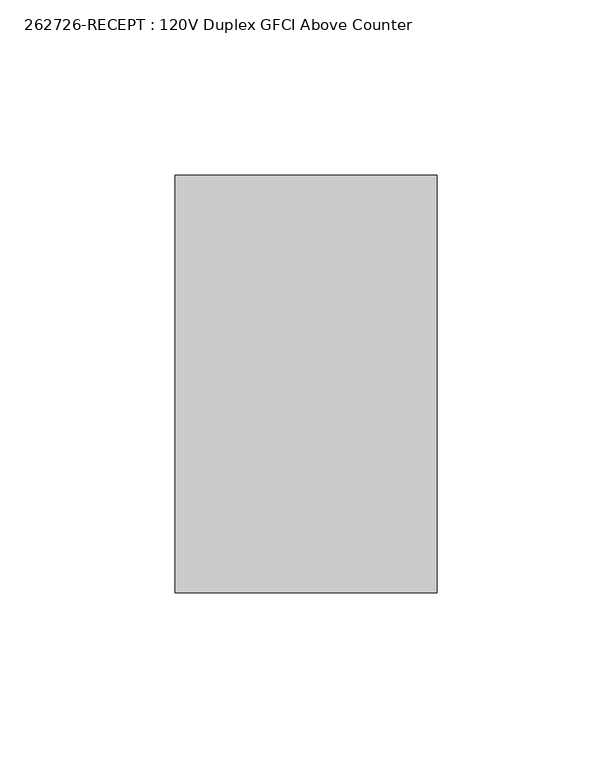
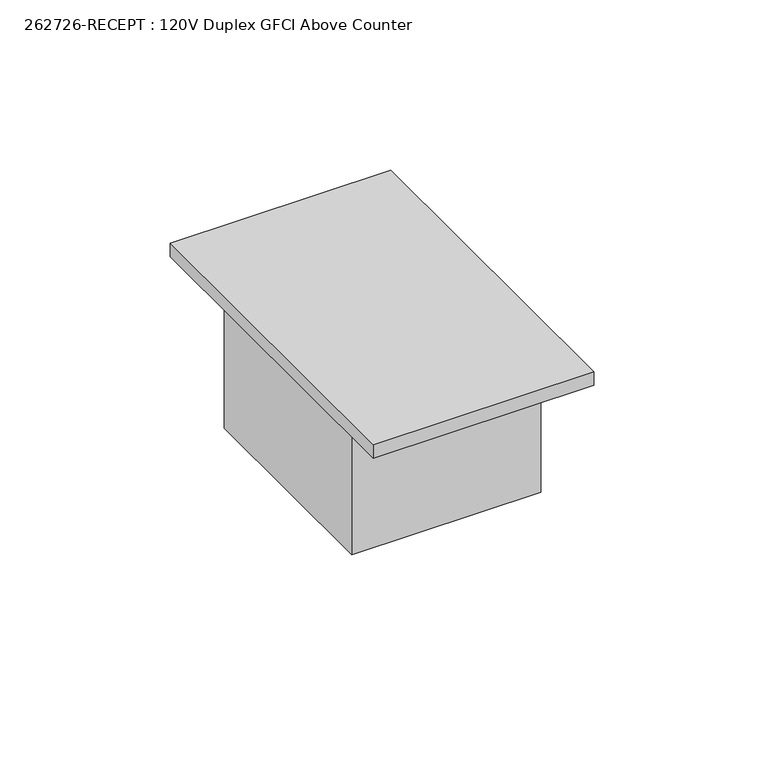
"""IFC4 building model written with IfcOpenShell, lengths in millimetres: proxy geometry, 262726-RECEPT : 120V Duplex GFCI Above Counter."""

from ifc_helpers import new_model, si_unit, frame, origin, origin_with_axes, place, context, project, spatial, polyline, outline, extrude, source, transform, mapped, element, save


def proxy_262726_recept_120v_duplex_gfci_above_counter_148ccacc(model_context):
    return source(origin(), model_context, "Body", "SweptSolid", [
        extrude(outline(polyline([(15.7308594, 59.5808594), (15.7308594, -59.5808594), (-58.9808594, -59.5808594), (-58.9808594, 59.5808594), (15.7308594, 59.5808594)])), origin_with_axes(), (0.0, 0.0, 1.0), 4.7625),
        extrude(outline(polyline([(10.5191406, 37.5), (10.5191406, -37.5), (-53.4808594, -37.5), (-53.4808594, 37.5), (10.5191406, 37.5)])), frame((0.0, 0.0, -50.0), z_axis=(0.0, 0.0, 1.0), x_axis=(1.0, 0.0, 0.0)), (0.0, 0.0, 1.0), 50.0),
    ])


if __name__ == "__main__":
    model = new_model("IFC4")
    model_context = context("Model", 3, world=origin())
    ifc_project = project(units=[si_unit("LENGTHUNIT", "METRE", prefix="MILLI")], contexts=[model_context])
    site = spatial("IfcSite", under=ifc_project)
    building = spatial("IfcBuilding", under=site)
    placement = place(None, origin())
    proxy_262726_recept_120v_duplex_gfci_above_counter_shape = proxy_262726_recept_120v_duplex_gfci_above_counter_148ccacc(model_context)
    element("IfcBuildingElementProxy", 1, Name="262726-RECEPT : 120V Duplex GFCI Above Counter", ObjectType="262726-RECEPT : 120V Duplex GFCI Above Counter", at=placement, inside=building, context=model_context, shape_type="MappedRepresentation", body=[
        mapped(proxy_262726_recept_120v_duplex_gfci_above_counter_shape, transform((0.0, 0.0, 0.0), x_axis=(1.0, 0.0, 0.0), y_axis=(0.0, 1.0, 0.0), z_axis=(0.0, 0.0, 1.0))),
    ])
    save(model, "model.ifc")

# Revit data of these elements
# Project information
#   Building Name = "RE1"
#   Client Name = "Client Name"
#   Project Address = "Project Address On One Line"
#   Project Name = "PROJECT NAME"
#   Project Number = "918741"
# Type "262726-RECEPT : 120V Duplex GFCI Above Counter"
#   MasterFormat = "26 27 26 Wiring Devices"
#   Model = "Generic"
#   Manufacturer = "Generic"
#   Label = "CT GFI"
#   Voltage = 120 V
#   Power Factor = 1
#   Phase = 1
#   Frequency = 60 Hz
#   Default Elevation = 1050 mm
#   Apparent Load = 180 VA
#   Show Label = yes
#   Number of Poles = 1
#   Anno Adjust [instance default] = no
#   Symbol = SYMBOL-Electrical : Receptacle Duplex GFCI
#   Receptacle = element 475861
#   Load Classification = Receptacle
#   Face Plate [instance default] = element 475865
#   Assembly Code = ""
